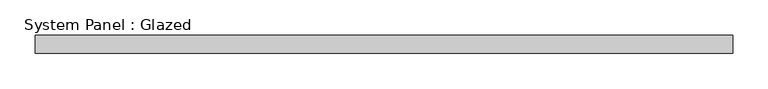
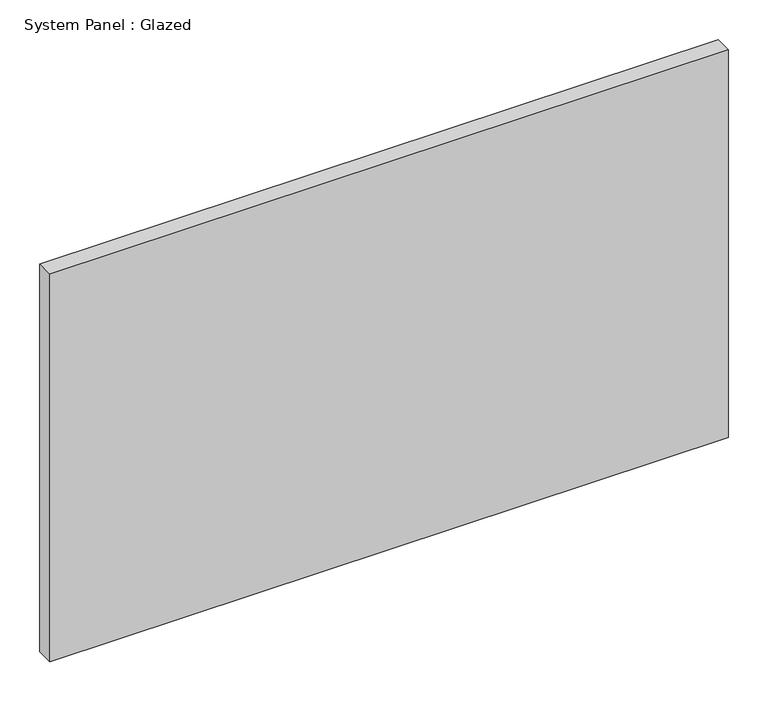
"""IFC4 building model written with IfcOpenShell, lengths in millimetres: plate geometry, System Panel : Glazed."""

from ifc_helpers import new_model, si_unit, origin, origin_with_axes, place, context, project, spatial, polyline, outline, extrude, source, transform, mapped, element, save


def system_panel_glazed_a77709dc(model_context):
    return source(origin(), model_context, "Body", "SweptSolid", [
        extrude(outline(polyline([(493.7595864, 19.05), (-493.7595864, 19.05), (-493.7595864, 44.45), (493.7595864, 44.45), (493.7595864, 19.05)])), origin_with_axes(), (0.0, 0.0, 1.0), 596.9),
    ])


if __name__ == "__main__":
    model = new_model("IFC4")
    model_context = context("Model", 3, world=origin())
    ifc_project = project(units=[si_unit("LENGTHUNIT", "METRE", prefix="MILLI")], contexts=[model_context])
    site = spatial("IfcSite", under=ifc_project)
    building = spatial("IfcBuilding", under=site)
    placement = place(None, origin())
    system_panel_glazed_shape = system_panel_glazed_a77709dc(model_context)
    element("IfcPlate", 1, ObjectType="System Panel : Glazed", at=placement, inside=building, context=model_context, shape_type="MappedRepresentation", body=[
        mapped(system_panel_glazed_shape, transform((0.0, 0.0, 0.0), x_axis=(1.0, 0.0, 0.0), y_axis=(0.0, 1.0, 0.0), z_axis=(0.0, 0.0, 1.0))),
    ])
    save(model, "model.ifc")

# Revit data of these elements
# Element 1 (IfcPlate, "System Panel : Glazed")
#   Materials on its faces: "Glass"
# Materials
#   "Glass": class "Glass", colour RGB 0 128 192, transparency 0.75
